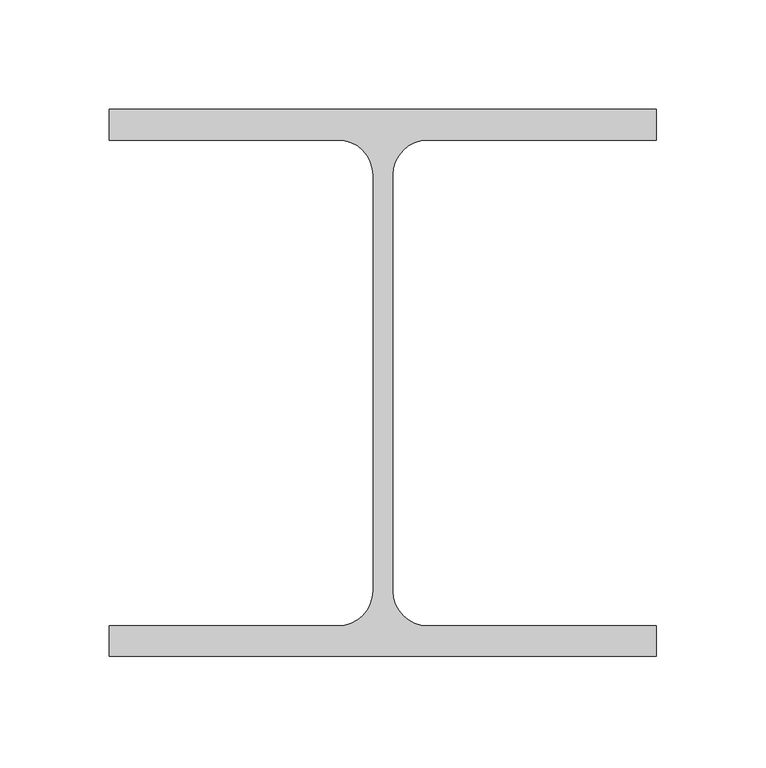
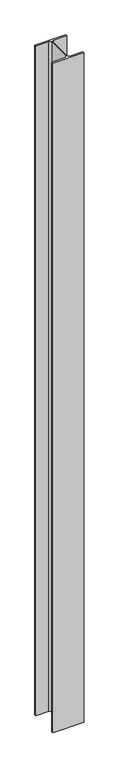
"""IFC4 building model written with IfcOpenShell, lengths in millimetres: column geometry, 0912_Steel Column_H_KSD3502 : H_SC_ASC_H-250x250x9x14."""

from ifc_helpers import new_model, si_unit, point, frame, frame_2d, origin, place, context, project, spatial, polyline, circle_curve, trimmed, segment, composite_curve, outline, extrude, source, transform, mapped, element, save


def column_6a202524(model_context):
    return source(origin(), model_context, "Body", "SweptSolid", [
        extrude(outline(composite_curve([segment(polyline([(125.0, 125.0), (125.0, 111.0), (20.5, 111.0)]), True, "CONTINUOUS"), segment(trimmed(circle_curve(frame_2d((20.5, 95.0)), 16.0), [point((20.5, 111.0))], [point((4.5, 95.0))], True, "CARTESIAN"), True, "CONTINUOUS"), segment(polyline([(4.5, 95.0), (4.5, -95.0)]), True, "CONTINUOUS"), segment(trimmed(circle_curve(frame_2d((20.5, -95.0)), 16.0), [point((4.5, -95.0))], [point((20.5, -111.0))], True, "CARTESIAN"), True, "CONTINUOUS"), segment(polyline([(20.5, -111.0), (125.0, -111.0), (125.0, -125.0), (-125.0, -125.0), (-125.0, -111.0), (-20.5, -111.0)]), True, "CONTINUOUS"), segment(trimmed(circle_curve(frame_2d((-20.5, -95.0)), 16.0), [point((-20.5, -111.0))], [point((-4.5, -95.0))], True, "CARTESIAN"), True, "CONTINUOUS"), segment(polyline([(-4.5, -95.0), (-4.5, 95.0)]), True, "CONTINUOUS"), segment(trimmed(circle_curve(frame_2d((-20.5, 95.0)), 16.0), [point((-4.5, 95.0))], [point((-20.5, 111.0))], True, "CARTESIAN"), True, "CONTINUOUS"), segment(polyline([(-20.5, 111.0), (-125.0, 111.0), (-125.0, 125.0), (125.0, 125.0)]), True, "CONTINUOUS")], self_intersect=False)), frame((0.0, 0.0, 599.9720055), z_axis=(0.0, 0.0, 1.0), x_axis=(1.0, 0.0, 0.0)), (0.0, 0.0, 1.0), 5700.0),
    ])


if __name__ == "__main__":
    model = new_model("IFC4")
    model_context = context("Model", 3, world=origin())
    ifc_project = project(units=[si_unit("LENGTHUNIT", "METRE", prefix="MILLI")], contexts=[model_context])
    site = spatial("IfcSite", under=ifc_project)
    building = spatial("IfcBuilding", under=site)
    placement = place(None, origin())
    column_shape = column_6a202524(model_context)
    element("IfcColumn", 1, ObjectType="0912_Steel Column_H_KSD3502 : H_SC_ASC_H-250x250x9x14", at=placement, inside=building, context=model_context, shape_type="MappedRepresentation", body=[
        mapped(column_shape, transform((0.0, 0.0, 0.0), x_axis=(1.0, 0.0, 0.0), y_axis=(0.0, 1.0, 0.0), z_axis=(0.0, 0.0, 1.0))),
    ])
    save(model, "model.ifc")

# Revit data of these elements
# Type "0912_Steel Column_H_KSD3502 : H_SC_ASC_H-250x250x9x14"
#   H_WM Code_1 = "S01AA002-00001 | Main Steel Structure Fabrication Work | Shelter/Building | Medium Steel - Standard (90KG/M>Weight≥30KG/M) | Material: (   )"
#   H_WM Code_2 = "S03AA028-00001 | Main Steel Structure Erection Work | Shelter/Building | Medium Steel (90KG/M>Weight≥30KG/M) | Material: (   )"
#   H_WM Code_3 = "S01AA010-00001 | Main Steel Structure Fabrication Work | Shelter/Building | Steel Painting/Coating | for Non-Fireproofed Steel Surface, Surface Preparation, Primer, Second & Final Coat | Material: (   )"
#   H_Q'ty Cal Type Tag = "SC-Q2"
#   Width = 25.0 cm
#   Web Thickness = 0.9 cm
#   Web Fillet = 1.6 cm
#   Warping Constant = 507646.0 cm⁶
#   Torsional Moment of Inertia = 51.4681 cm⁴
#   Section Area = 92.18 cm²
#   Plastic Modulus weak axis = 444.0 cm³
#   Plastic Modulus strong axis = 960.0 cm³
#   Perimeter = 1.46 m²/m
#   Nominal Weight = 72.40 kgf/m
#   Moment of Inertia weak axis = 3650.00 cm⁴
#   Moment of Inertia strong axis = 10800.00 cm⁴
#   Height = 25.0 cm
#   Flange Thickness = 1.4 cm
#   Elastic Modulus weak axis = 292.0 cm³
#   Elastic Modulus strong axis = 867.0 cm³
#   Centroid Vertical = 12.5 cm
#   Centroid Horizontal = 12.5 cm
#   Structural Material [instance default] = Steel, 45-345
#   Section Name Key = ""
#   Bolt Spacing = 0
#   Assembly Code = ""
# Element 1 (IfcColumn, "0912_Steel Column_H_KSD3502 : H_SC_ASC_H-250x250x9x14")
#   Structural Material = A03AD029-00005_Anchor Bolt (Installation only)_M24
#   Materials on its faces: "A03AD029-00005_Anchor Bolt (Installation only)_M24"
# Materials
#   "Steel, 45-345": class "Metal", colour RGB 189 187 185, transparency 0, Description = "Steel 345 MPa", Cost = 0
#   "A03AD029-00005_Anchor Bolt (Installation only)_M24": class "Unassigned", colour RGB 84 83 81, transparency 0, Cost = 0
